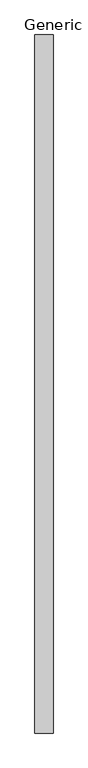
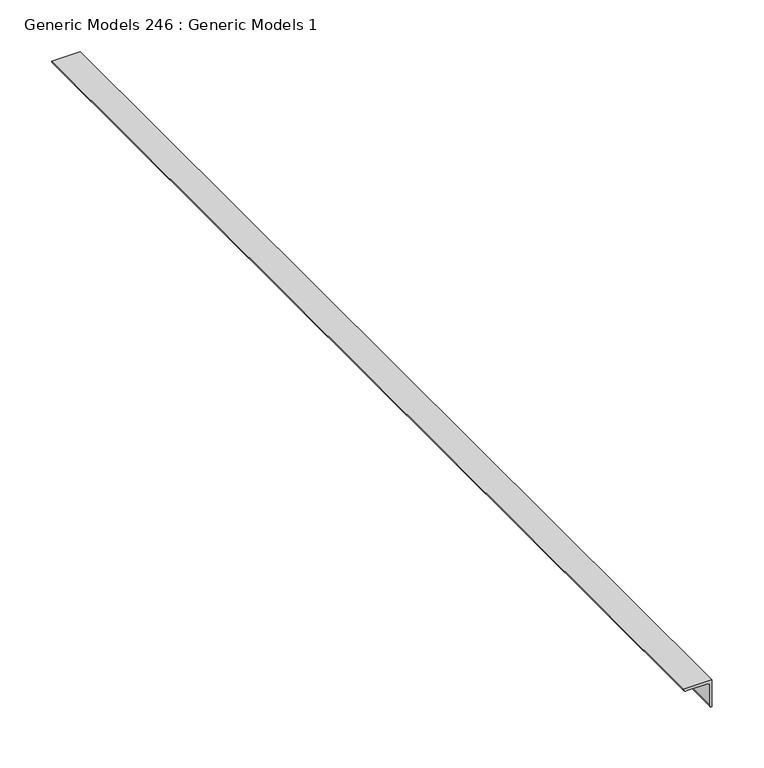
"""IFC4 building model written with IfcOpenShell, lengths in millimetres: proxy geometry, Generic Models 246 : Generic Models 1."""

from ifc_helpers import new_model, si_unit, point, frame, frame_2d, origin, place, context, project, spatial, polyline, circle_curve, trimmed, segment, composite_curve, outline, extrude, source, transform, mapped, element, save


def generic_models_246_generic_models_1_33f707d8(model_context):
    return source(origin(), model_context, "Body", "SweptSolid", [
        extrude(outline(composite_curve([segment(polyline([(4267.2, 47363.0625), (4267.2, 47331.3125)]), True, "CONTINUOUS"), segment(trimmed(circle_curve(frame_2d((4267.2, 47334.4875)), 3.175), [point((4267.2, 47331.3125))], [point((4264.025, 47334.4875))], False, "CARTESIAN"), True, "CONTINUOUS"), segment(polyline([(4264.025, 47334.4875), (4264.025, 47358.3)]), True, "CONTINUOUS"), segment(trimmed(circle_curve(frame_2d((4262.4375, 47358.3)), 1.5875), [point((4264.025, 47358.3))], [point((4262.4375, 47359.8875))], True, "CARTESIAN"), True, "CONTINUOUS"), segment(polyline([(4262.4375, 47359.8875), (4238.625, 47359.8875)]), True, "CONTINUOUS"), segment(trimmed(circle_curve(frame_2d((4238.625, 47363.0625)), 3.175), [point((4238.625, 47359.8875))], [point((4235.45, 47363.0625))], False, "CARTESIAN"), True, "CONTINUOUS"), segment(polyline([(4235.45, 47363.0625), (4267.2, 47363.0625)]), True, "CONTINUOUS")], self_intersect=False)), frame((0.0, 0.0, 0.0), z_axis=(0.0, 1.0, 0.0), x_axis=(0.0, 0.0, 1.0)), (0.0, 0.0, 1.0), 1219.2),
    ])


if __name__ == "__main__":
    model = new_model("IFC4")
    model_context = context("Model", 3, world=origin())
    ifc_project = project(units=[si_unit("LENGTHUNIT", "METRE", prefix="MILLI")], contexts=[model_context])
    site = spatial("IfcSite", under=ifc_project)
    building = spatial("IfcBuilding", under=site)
    placement = place(None, origin())
    generic_models_246_generic_models_1_shape = generic_models_246_generic_models_1_33f707d8(model_context)
    element("IfcBuildingElementProxy", 1, Name="Generic Models 246 : Generic Models 1", ObjectType="Generic Models 246 : Generic Models 1", at=placement, inside=building, context=model_context, shape_type="MappedRepresentation", body=[
        mapped(generic_models_246_generic_models_1_shape, transform((0.0, 0.0, 0.0), x_axis=(1.0, 0.0, 0.0), y_axis=(0.0, 1.0, 0.0), z_axis=(0.0, 0.0, 1.0))),
    ])
    save(model, "model.ifc")

# Revit data of these elements
# Element 1 (IfcBuildingElementProxy, "Generic Models 246 : Generic Models 1")
#   Materials on its faces: "BULKHEAD FRAME WORK"
# Materials
#   "BULKHEAD FRAME WORK": class "Metal", colour RGB 189 187 185, transparency 0, Description = "Structural steel 50ksi", Cost = 0
